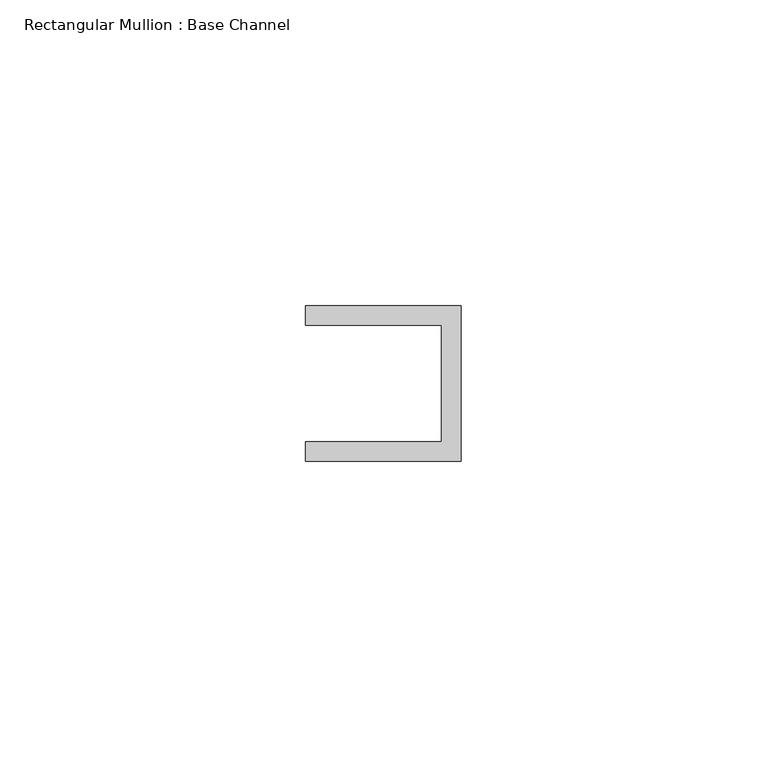
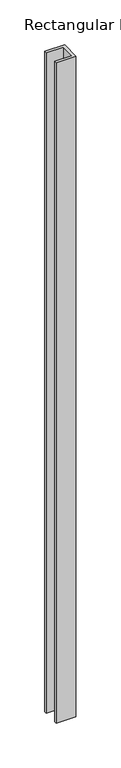
"""IFC4 building model written with IfcOpenShell, lengths in millimetres: member geometry, Rectangular Mullion : Base Channel."""

from ifc_helpers import new_model, si_unit, frame, origin, place, context, project, spatial, polyline, outline, extrude, source, transform, mapped, element, save


def rectangular_mullion_base_channel_ed4b310c(model_context):
    return source(origin(), model_context, "Body", "SweptSolid", [
        extrude(outline(polyline([(0.0, -12.7), (-25.4, -12.7), (-25.4, -9.525), (-3.175, -9.525), (-3.175, 9.525), (-25.4, 9.525), (-25.4, 12.7), (0.0, 12.7), (0.0, -12.7)])), frame((0.0, 0.0, -900.1125), z_axis=(0.0, 0.0, 1.0), x_axis=(1.0, 0.0, 0.0)), (0.0, 0.0, 1.0), 900.1125),
    ])


if __name__ == "__main__":
    model = new_model("IFC4")
    model_context = context("Model", 3, world=origin())
    ifc_project = project(units=[si_unit("LENGTHUNIT", "METRE", prefix="MILLI")], contexts=[model_context])
    site = spatial("IfcSite", under=ifc_project)
    building = spatial("IfcBuilding", under=site)
    placement = place(None, origin())
    rectangular_mullion_base_channel_shape = rectangular_mullion_base_channel_ed4b310c(model_context)
    element("IfcMember", 1, ObjectType="Rectangular Mullion : Base Channel", at=placement, inside=building, context=model_context, shape_type="MappedRepresentation", body=[
        mapped(rectangular_mullion_base_channel_shape, transform((0.0, 0.0, 0.0), x_axis=(1.0, 0.0, 0.0), y_axis=(0.0, 1.0, 0.0), z_axis=(0.0, 0.0, 1.0))),
    ])
    save(model, "model.ifc")

# Revit data of these elements
# Type "Rectangular Mullion : Base Channel"
#   built-in parameter 1007322 = 0.0833333 (stored number, unit not read)
#   built-in parameter 1007321 = 0.0416667 (stored number, unit not read)
#   built-in parameter 1007320 = -0.03125 (stored number, unit not read)
# Element 1 (IfcMember, "Rectangular Mullion : Base Channel")
#   Materials on its faces: "ALUM"
# Materials
#   "ALUM": class "Generic", colour RGB 157 157 157, transparency 0, Cost = 0
